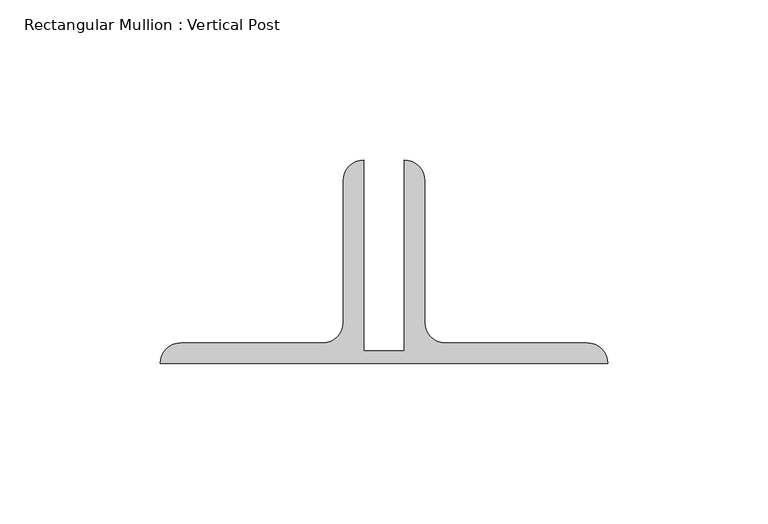
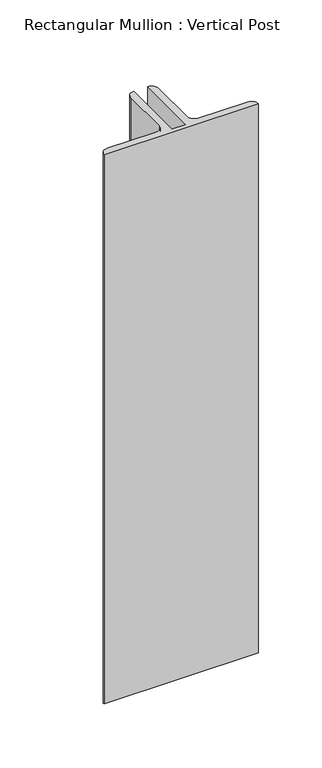
"""IFC4 building model written with IfcOpenShell, lengths in millimetres: member geometry, Rectangular Mullion : Vertical Post."""

from ifc_helpers import new_model, si_unit, point, frame, frame_2d, origin, place, context, project, spatial, polyline, circle_curve, trimmed, segment, composite_curve, outline, extrude, source, transform, mapped, element, save


def rectangular_mullion_vertical_post_01d6e3cf(model_context):
    return source(origin(), model_context, "Body", "SweptSolid", [
        extrude(outline(composite_curve([segment(polyline([(-63.5, 22.9145205), (-63.5, 82.55)]), True, "CONTINUOUS"), segment(trimmed(circle_curve(frame_2d((-63.5, 76.2)), 6.35), [point((-63.5, 82.55))], [point((-57.15, 76.2))], False, "CARTESIAN"), True, "CONTINUOUS"), segment(polyline([(-57.15, 76.2), (-57.15, 31.75)]), True, "CONTINUOUS"), segment(trimmed(circle_curve(frame_2d((-50.8, 31.75)), 6.35), [point((-57.15, 31.75))], [point((-50.8, 25.4))], True, "CARTESIAN"), True, "CONTINUOUS"), segment(polyline([(-50.8, 25.4), (-6.35, 25.4)]), True, "CONTINUOUS"), segment(trimmed(circle_curve(frame_2d((-6.35, 19.05)), 6.35), [point((-6.35, 25.4))], [point((0.0, 19.05))], False, "CARTESIAN"), True, "CONTINUOUS"), segment(polyline([(0.0, 19.05), (-139.7, 19.05)]), True, "CONTINUOUS"), segment(trimmed(circle_curve(frame_2d((-133.35, 19.05)), 6.35), [point((-139.7, 19.05))], [point((-133.35, 25.4))], False, "CARTESIAN"), True, "CONTINUOUS"), segment(polyline([(-133.35, 25.4), (-88.9, 25.4)]), True, "CONTINUOUS"), segment(trimmed(circle_curve(frame_2d((-88.9, 31.75)), 6.35), [point((-88.9, 25.4))], [point((-82.55, 31.75))], True, "CARTESIAN"), True, "CONTINUOUS"), segment(polyline([(-82.55, 31.75), (-82.55, 76.2)]), True, "CONTINUOUS"), segment(trimmed(circle_curve(frame_2d((-76.2, 76.2)), 6.35), [point((-82.55, 76.2))], [point((-76.2, 82.55))], False, "CARTESIAN"), True, "CONTINUOUS"), segment(polyline([(-76.2, 82.55), (-76.2, 22.9145205), (-63.5, 22.9145205)]), True, "CONTINUOUS")], self_intersect=False)), frame((0.0, 0.0, -526.8889998), z_axis=(0.0, 0.0, 1.0), x_axis=(1.0, 0.0, 0.0)), (0.0, 0.0, 1.0), 526.8889998),
    ])


if __name__ == "__main__":
    model = new_model("IFC4")
    model_context = context("Model", 3, world=origin())
    ifc_project = project(units=[si_unit("LENGTHUNIT", "METRE", prefix="MILLI")], contexts=[model_context])
    site = spatial("IfcSite", under=ifc_project)
    building = spatial("IfcBuilding", under=site)
    placement = place(None, origin())
    rectangular_mullion_vertical_post_shape = rectangular_mullion_vertical_post_01d6e3cf(model_context)
    element("IfcMember", 1, ObjectType="Rectangular Mullion : Vertical Post", at=placement, inside=building, context=model_context, shape_type="MappedRepresentation", body=[
        mapped(rectangular_mullion_vertical_post_shape, transform((0.0, 0.0, 0.0), x_axis=(1.0, 0.0, 0.0), y_axis=(0.0, 1.0, 0.0), z_axis=(0.0, 0.0, 1.0))),
    ])
    save(model, "model.ifc")

# Revit data of these elements
# Type "Rectangular Mullion : Vertical Post"
#   built-in parameter 1007351 = -0.0625 (stored number, unit not read)
#   built-in parameter 1007322 = 0.0126789 (stored number, unit not read)
#   built-in parameter 1007321 = 0.229167 (stored number, unit not read)
#   built-in parameter 1007320 = 0.229167 (stored number, unit not read)
# Element 1 (IfcMember, "Rectangular Mullion : Vertical Post")
#   Materials on its faces: "GATE POST: (2) BACK/BACK GALVANIZED ANGLES"
# Materials
#   "GATE POST: (2) BACK/BACK GALVANIZED ANGLES": class "Unassigned", colour RGB 211 211 211, transparency 0, Cost = 0
